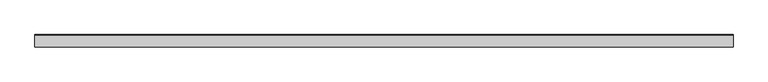
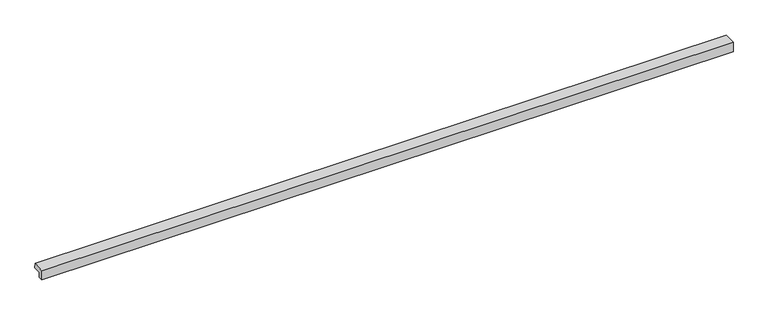
"""IFC4 building model written with IfcOpenShell, lengths in millimetres: proxy geometry, Inner panel:Inner panel:1:Inner panel:1 : Inner panel:Inner panel:300324:2:Inner panel:1:Inner panel:1 : Inner panel:Inner panel:300324:2 : Inner panel:Inner panel:1:Inner panel:1 : Inner panel:Inner panel:300324:300043:10 : Inner panel:Inner panel:1:Inner panel:1 : Inner panel:Inner panel:300324:2:Inner panel:1:Inner panel:1 : Inner panel:Inner panel:300324:2 : Inner panel:Inner panel:1:Inner panel:1 : Inner panel:Inner panel:300324:300043:308120."""

from ifc_helpers import new_model, si_unit, frame, origin, place, context, project, spatial, polyline, outline, extrude, source, transform, mapped, element, save


def generic_models_48d54057(model_context):
    return source(origin(), model_context, "Body", "SweptSolid", [
        extrude(outline(polyline([(-536469.513904, 10161.2521589), (-536468.1912252, 10129.5078678), (-536521.0312005, 10127.3062022), (-536521.0312005, 10088.6481152), (-536553.5329071, 10088.6481152), (-536553.5329071, 10157.7513671), (-536469.513904, 10161.2521589)])), frame((591306.0367242, 0.0, 0.0), z_axis=(1.0, 0.0, 0.0), x_axis=(0.0, 1.0, 0.0)), (0.0, 0.0, 1.0), 4876.8),
    ])


if __name__ == "__main__":
    model = new_model("IFC4")
    model_context = context("Model", 3, world=origin())
    ifc_project = project(units=[si_unit("LENGTHUNIT", "METRE", prefix="MILLI")], contexts=[model_context])
    site = spatial("IfcSite", under=ifc_project)
    building = spatial("IfcBuilding", under=site)
    placement = place(None, origin())
    generic_models_shape = generic_models_48d54057(model_context)
    element("IfcBuildingElementProxy", 1, Name="Inner panel:Inner panel:1:Inner panel:1 : Inner panel:Inner panel:300324:2:Inner panel:1:Inner panel:1 : Inner panel:Inner panel:300324:2 : Inner panel:Inner panel:1:Inner panel:1 : Inner panel:Inner panel:300324:300043:10 : Inner panel:Inner panel:1:Inner panel:1 : Inner panel:Inner panel:300324:2:Inner panel:1:Inner panel:1 : Inner panel:Inner panel:300324:2 : Inner panel:Inner panel:1:Inner panel:1 : Inner panel:Inner panel:300324:300043:308120", ObjectType="Inner panel:Inner panel:1:Inner panel:1 : Inner panel:Inner panel:300324:2:Inner panel:1:Inner panel:1 : Inner panel:Inner panel:300324:2 : Inner panel:Inner panel:1:Inner panel:1 : Inner panel:Inner panel:300324:300043:10 : Inner panel:Inner panel:1:Inner panel:1 : Inner panel:Inner panel:300324:2:Inner panel:1:Inner panel:1 : Inner panel:Inner panel:300324:2 : Inner panel:Inner panel:1:Inner panel:1 : Inner panel:Inner panel:300324:300043:308120", at=placement, inside=building, context=model_context, shape_type="MappedRepresentation", body=[
        mapped(generic_models_shape, transform((0.0, 0.0, 0.0), x_axis=(1.0, 0.0, 0.0), y_axis=(0.0, 1.0, 0.0), z_axis=(0.0, 0.0, 1.0))),
    ])
    save(model, "model.ifc")

# Revit data of these elements
# Type "Inner panel:Inner panel:1:Inner panel:1 : Inner panel:Inner panel:300324:2:Inner panel:1:Inner panel:1 : Inner panel:Inner panel:300324:2 : Inner panel:Inner panel:1:Inner panel:1 : Inner panel:Inner panel:300324:300043:10 : Inner panel:Inner panel:1:Inner panel:1 : Inner panel:Inner panel:300324:2:Inner panel:1:Inner panel:1 : Inner panel:Inner panel:300324:2 : Inner panel:Inner panel:1:Inner panel:1 : Inner panel:Inner panel:300324:300043:308120"
#   NameOverride = "Inner panel:Inner panel:1:Inner panel:1 : Inner panel:Inner panel:300324:2:Inner panel:1:Inner panel:1 : Inner panel:Inner panel:300324:2 : Inner panel:Inner panel:1:Inner panel:1 : Inner panel:Inner panel:300324:300043:308120"
#   ObjectTypeOverride = "Inner panel:1:Inner panel:1 : Inner panel:Inner panel:300324:2 : Inner panel:Inner panel:1:Inner panel:1 : Inner panel:Inner panel:300324:300043"
#   Reference = "Inner panel"
#   Tag = "308120"
# Element 1 (IfcBuildingElementProxy, "Inner panel:Inner panel:1:Inner panel:1 : Inner panel:Inner panel:300324:2:Inner panel:1:Inner panel:1 : Inner panel:Inner panel:300324:2 : Inner panel:Inner panel:1:Inner panel:1 : Inner panel:Inner panel:300324:300043:10 : Inner panel:Inner panel:1:Inner panel:1 : Inner panel:Inner panel:300324:2:Inner panel:1:Inner panel:1 : Inner panel:Inner panel:300324:2 : Inner panel:Inner panel:1:Inner panel:1 : Inner panel:Inner panel:300324:300043:308120")
#   Materials on its faces: "LOW VOLUMN EXPANDABLE FOAM INSULATION"
# Materials
#   "LOW VOLUMN EXPANDABLE FOAM INSULATION": class "Unassigned", colour RGB 213 216 95, transparency 0, Cost = 0
